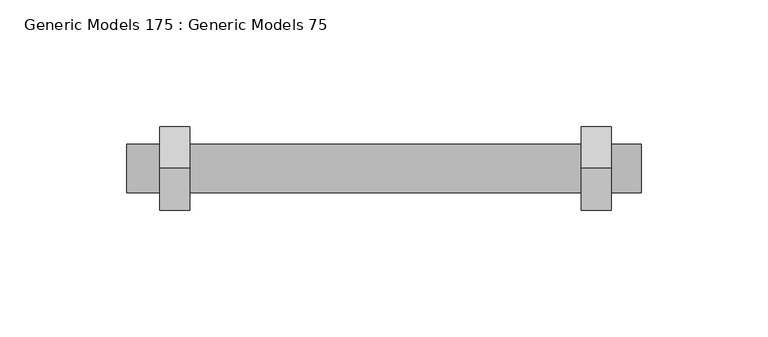
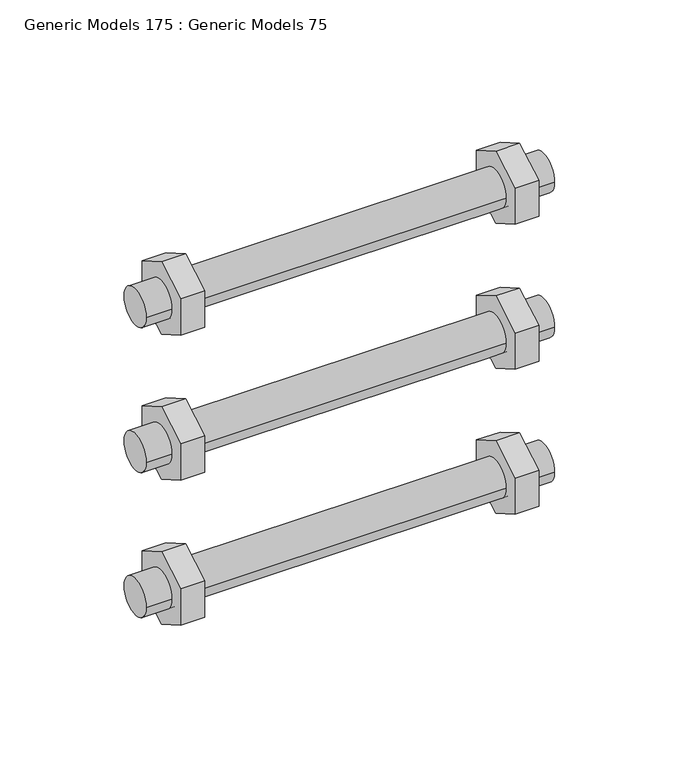
"""IFC4 building model written with IfcOpenShell, lengths in millimetres: proxy geometry, Generic Models 175 : Generic Models 75."""

import ifcopenshell
import ifcopenshell.guid

model = None  # the IFC model being written
_history = None  # IfcOwnerHistory: only IFC2X3 demands one
_inside = {}  # id of a spatial element -> (the spatial element, [elements in it])
_under = {}  # id of a project, library or spatial element -> (it, [spatial elements below it])
_declared = {}  # id of a project -> (the project, [libraries it declares])
_typed = {}  # id of a type object -> (the type object, [elements of that type])
_made_of = {}  # id of a material, layer set ... -> (it, [elements and type objects made of it])


def new_model(schema):
    """Start an empty IFC model of exactly this schema.

    Asked for "IFC4X3", IfcOpenShell would pick the latest addendum, in which some entities
    have other attributes; the version numbers below select the first issue.
    IFC2X3 requires an IfcOwnerHistory on every rooted entity: one is made here for all.
    """
    global model, _history
    if schema == "IFC4X3":
        model = ifcopenshell.file(schema_version=(4, 3, 0, 0))
    else:
        model = ifcopenshell.file(schema=schema)
    _inside.clear()
    _under.clear()
    _declared.clear()
    _typed.clear()
    _made_of.clear()
    _history = None
    if model.schema == "IFC2X3":
        org = make("IfcOrganization", Name="unknown")
        user = make(
            "IfcPersonAndOrganization",
            ThePerson=make("IfcPerson", FamilyName="unknown"),
            TheOrganization=org,
        )
        app = make(
            "IfcApplication",
            ApplicationDeveloper=org,
            Version="unknown",
            ApplicationFullName="unknown",
            ApplicationIdentifier="unknown",
        )
        _history = make(
            "IfcOwnerHistory",
            OwningUser=user,
            OwningApplication=app,
            ChangeAction="ADDED",
            CreationDate=0,
        )
    return model


def make(cls, **values):
    """One entity of the class cls with the attributes given. An attribute that is None is left unset."""
    return model.create_entity(
        cls, **{name: value for name, value in values.items() if value is not None}
    )


def rooted(cls, **values):
    """An entity with a GlobalId (a new one), such as an element, a storey or a relation."""
    return make(cls, GlobalId=ifcopenshell.guid.new(), OwnerHistory=_history, **values)


def si_unit(unit_type, name, prefix=None):
    """IfcSIUnit, for example si_unit("LENGTHUNIT", "METRE", prefix="MILLI")."""
    return make("IfcSIUnit", UnitType=unit_type, Prefix=prefix, Name=name)


def assignment(units):
    """IfcUnitAssignment: the units of a project."""
    return None if units is None else make("IfcUnitAssignment", Units=units)


def point(xyz):
    """IfcCartesianPoint."""
    return None if xyz is None else make("IfcCartesianPoint", Coordinates=xyz)


def direction(xyz):
    """IfcDirection."""
    return None if xyz is None else make("IfcDirection", DirectionRatios=xyz)


def frame(location, z_axis=None, x_axis=None):
    """IfcAxis2Placement3D, a coordinate frame: its origin and axes. An axis left out is left unset."""
    return make(
        "IfcAxis2Placement3D",
        Location=point(location),
        Axis=direction(z_axis),
        RefDirection=direction(x_axis),
    )


def frame_2d(location, x_axis=None):
    """IfcAxis2Placement2D, a coordinate frame in the plane: its origin and x axis."""
    return make(
        "IfcAxis2Placement2D", Location=point(location), RefDirection=direction(x_axis)
    )


def origin():
    """The frame at (0, 0, 0) with its axes left unset."""
    return frame((0.0, 0.0, 0.0))


def place(relative_to, where):
    """IfcLocalPlacement: puts the frame where relative to a parent placement (None: the world)."""
    return make(
        "IfcLocalPlacement", PlacementRelTo=relative_to, RelativePlacement=where
    )


def context(
    kind, dimensions, precision=None, world=None, true_north=None, identifier=None
):
    """IfcGeometricRepresentationContext, for example the 3D "Model" context."""
    return make(
        "IfcGeometricRepresentationContext",
        ContextIdentifier=identifier,
        ContextType=kind,
        CoordinateSpaceDimension=dimensions,
        Precision=precision,
        WorldCoordinateSystem=world,
        TrueNorth=true_north,
    )


def project(units=None, contexts=None):
    """IfcProject with its units and contexts."""
    return rooted(
        "IfcProject",
        Name="project",
        RepresentationContexts=contexts,
        UnitsInContext=assignment(units),
    )


def spatial(cls, under=None, at=None, **own):
    """A site, building, storey or space (cls), placed at a placement, below another one or the project."""
    s = rooted(cls, ObjectPlacement=at, **own)
    if under is not None:
        _under.setdefault(under.id(), (under, []))[1].append(s)
    return s


def polyline(points):
    """IfcPolyline through the points."""
    return make("IfcPolyline", Points=[point(p) for p in points])


def circle_curve(where, radius):
    """IfcCircle in the frame where."""
    return make("IfcCircle", Position=where, Radius=radius)


def trimmed(basis, trim1, trim2, sense, master):
    """IfcTrimmedCurve: the piece of a basis curve between two trims."""
    return make(
        "IfcTrimmedCurve",
        BasisCurve=basis,
        Trim1=trim1,
        Trim2=trim2,
        SenseAgreement=sense,
        MasterRepresentation=master,
    )


def segment(curve, same_sense, transition):
    """IfcCompositeCurveSegment."""
    return make(
        "IfcCompositeCurveSegment",
        Transition=transition,
        SameSense=same_sense,
        ParentCurve=curve,
    )


def composite_curve(segments, self_intersect=None):
    """IfcCompositeCurve: segments joined end to end."""
    return make("IfcCompositeCurve", Segments=segments, SelfIntersect=self_intersect)


def outline(outer, holes=None, kind="AREA"):
    """IfcArbitraryClosedProfileDef: a profile drawn as a closed curve; with holes, ...WithVoids."""
    if holes is None:
        return make("IfcArbitraryClosedProfileDef", ProfileType=kind, OuterCurve=outer)
    return make(
        "IfcArbitraryProfileDefWithVoids",
        ProfileType=kind,
        OuterCurve=outer,
        InnerCurves=holes,
    )


def extrude(swept, where, along, depth):
    """IfcExtrudedAreaSolid: the profile swept, set in the frame where, extruded along a direction by depth."""
    return make(
        "IfcExtrudedAreaSolid",
        SweptArea=swept,
        Position=where,
        ExtrudedDirection=direction(along),
        Depth=depth,
    )


def shape(context_of_items, identifier, shape_type, items):
    """IfcShapeRepresentation: the items that make up one representation, for example the "Body"."""
    return make(
        "IfcShapeRepresentation",
        ContextOfItems=context_of_items,
        RepresentationIdentifier=identifier,
        RepresentationType=shape_type,
        Items=items,
    )


def source(mapping_origin, context_of_items, identifier, shape_type, items):
    """IfcRepresentationMap: a shape defined once, which mapped items show again and again."""
    return make(
        "IfcRepresentationMap",
        MappingOrigin=mapping_origin,
        MappedRepresentation=shape(context_of_items, identifier, shape_type, items),
    )


def transform(
    local_origin,
    x_axis=None,
    y_axis=None,
    z_axis=None,
    scale=None,
    scale2=None,
    scale3=None,
    uniform=True,
):
    """IfcCartesianTransformationOperator3D, or its non-uniform kind. x_axis, y_axis, z_axis: its Axis1, 2, 3."""
    if uniform:
        return make(
            "IfcCartesianTransformationOperator3D",
            Axis1=direction(x_axis),
            Axis2=direction(y_axis),
            LocalOrigin=point(local_origin),
            Scale=scale,
            Axis3=direction(z_axis),
        )
    return make(
        "IfcCartesianTransformationOperator3DnonUniform",
        Axis1=direction(x_axis),
        Axis2=direction(y_axis),
        LocalOrigin=point(local_origin),
        Scale=scale,
        Axis3=direction(z_axis),
        Scale2=scale2,
        Scale3=scale3,
    )


def mapped(mapping_source, mapping_target):
    """IfcMappedItem: shows the shape of a source again, moved by a transform."""
    return make(
        "IfcMappedItem", MappingSource=mapping_source, MappingTarget=mapping_target
    )


def made_of(thing, what):
    """Note that an element or type object is made of a material, layer set ...; save() writes the relation."""
    if what is not None:
        _made_of.setdefault(what.id(), (what, []))[1].append(thing)
    return thing


def element(
    cls,
    number,
    at=None,
    inside=None,
    cuts=None,
    type_object=None,
    material=None,
    context=None,
    identifier="Body",
    shape_type=None,
    held_by="IfcProductDefinitionShape",
    body=None,
    shapes=None,
    **own,
):
    """One element of the class cls, such as IfcWall. Its Tag is "e" and its number.

    at: its placement. inside: the storey or other place that contains it. cuts: it is an
    opening in that element (IfcRelVoidsElement). A single representation is given by context,
    identifier, shape_type and body (its items); several are given by shapes. held_by: the class
    of the entity that holds the representations. save() writes the other relations.
    """
    e = rooted(cls, Tag="e%d" % number, ObjectPlacement=at, **own)
    if body is not None:
        shapes = [shape(context, identifier, shape_type, body)]
    if shapes is not None:
        e.Representation = make(held_by, Representations=shapes)
    if inside is not None:
        _inside.setdefault(inside.id(), (inside, []))[1].append(e)
    if cuts is not None:
        rooted(
            "IfcRelVoidsElement", RelatingBuildingElement=cuts, RelatedOpeningElement=e
        )
    if type_object is not None:
        _typed.setdefault(type_object.id(), (type_object, []))[1].append(e)
    return made_of(e, material)


def aggregate(whole, parts):
    """IfcRelAggregates: a whole, such as a stair, and the parts it consists of."""
    return rooted("IfcRelAggregates", RelatingObject=whole, RelatedObjects=parts)


def save(model, path):
    """Write the relations noted so far, then the file.

    IfcRelAggregates (storeys below a building ...), IfcRelContainedInSpatialStructure (elements
    in a storey), IfcRelDefinesByType, IfcRelAssociatesMaterial and IfcRelDeclares: one each for
    every whole, place, type object, material and project.
    """
    for whole, parts in _under.values():
        aggregate(whole, parts)
    for where, things in _inside.values():
        rooted(
            "IfcRelContainedInSpatialStructure",
            RelatedElements=things,
            RelatingStructure=where,
        )
    for kind, things in _typed.values():
        rooted("IfcRelDefinesByType", RelatedObjects=things, RelatingType=kind)
    for what, things in _made_of.values():
        rooted("IfcRelAssociatesMaterial", RelatedObjects=things, RelatingMaterial=what)
    for by, libraries in _declared.values():
        rooted("IfcRelDeclares", RelatingContext=by, RelatedDefinitions=libraries)
    model.write(path)


def generic_models_175_generic_models_75_7ebaa3f2(model_context):
    return source(origin(), model_context, "Body", "SweptSolid", [
        extrude(outline(polyline([(30896.7491273, 271852.097122), (30913.2469112, 271861.622122), (30929.7446951, 271852.097122), (30929.7446951, 271833.047122), (30913.2469112, 271823.522122), (30896.7491273, 271833.047122), (30896.7491273, 271852.097122)])), frame((31918.2596032, 0.0, 0.0), z_axis=(1.0, 0.0, 0.0), x_axis=(0.0, 1.0, 0.0)), (0.0, 0.0, 1.0), 11.90625),
        extrude(outline(polyline([(30896.7491273, 271775.897122), (30913.2469112, 271785.422122), (30929.7446951, 271775.897122), (30929.7446951, 271756.847122), (30913.2469112, 271747.322122), (30896.7491273, 271756.847122), (30896.7491273, 271775.897122)])), frame((31918.2596032, 0.0, 0.0), z_axis=(1.0, 0.0, 0.0), x_axis=(0.0, 1.0, 0.0)), (0.0, 0.0, 1.0), 11.90625),
        extrude(outline(polyline([(30896.7491273, 271699.697122), (30913.2469112, 271709.222122), (30929.7446951, 271699.697122), (30929.7446951, 271680.647122), (30913.2469112, 271671.122122), (30896.7491273, 271680.647122), (30896.7491273, 271699.697122)])), frame((31918.2596032, 0.0, 0.0), z_axis=(1.0, 0.0, 0.0), x_axis=(0.0, 1.0, 0.0)), (0.0, 0.0, 1.0), 11.90625),
        extrude(outline(polyline([(30896.7491273, 271852.097122), (30913.2469112, 271861.622122), (30929.7446951, 271852.097122), (30929.7446951, 271833.047122), (30913.2469112, 271823.522122), (30896.7491273, 271833.047122), (30896.7491273, 271852.097122)])), frame((31751.9689782, 0.0, 0.0), z_axis=(1.0, 0.0, 0.0), x_axis=(0.0, 1.0, 0.0)), (0.0, 0.0, 1.0), 11.90625),
        extrude(outline(polyline([(30896.7491273, 271775.897122), (30913.2469112, 271785.422122), (30929.7446951, 271775.897122), (30929.7446951, 271756.847122), (30913.2469112, 271747.322122), (30896.7491273, 271756.847122), (30896.7491273, 271775.897122)])), frame((31751.9689782, 0.0, 0.0), z_axis=(1.0, 0.0, 0.0), x_axis=(0.0, 1.0, 0.0)), (0.0, 0.0, 1.0), 11.90625),
        extrude(outline(polyline([(30896.7491273, 271699.697122), (30913.2469112, 271709.222122), (30929.7446951, 271699.697122), (30929.7446951, 271680.647122), (30913.2469112, 271671.122122), (30896.7491273, 271680.647122), (30896.7491273, 271699.697122)])), frame((31751.9689782, 0.0, 0.0), z_axis=(1.0, 0.0, 0.0), x_axis=(0.0, 1.0, 0.0)), (0.0, 0.0, 1.0), 11.90625),
        extrude(outline(composite_curve([segment(trimmed(circle_curve(frame_2d((30913.2469112, 271766.372122)), 9.525), [point((30922.7719112, 271766.372122))], [point((30903.7219112, 271766.372122))], False, "CARTESIAN"), True, "CONTINUOUS"), segment(trimmed(circle_curve(frame_2d((30913.2469112, 271766.372122)), 9.525), [point((30903.7219112, 271766.372122))], [point((30922.7719112, 271766.372122))], False, "CARTESIAN"), True, "CONTINUOUS")], self_intersect=False)), frame((31738.8721032, 0.0, 0.0), z_axis=(1.0, 0.0, 0.0), x_axis=(0.0, 1.0, 0.0)), (0.0, 0.0, 1.0), 203.2),
        extrude(outline(composite_curve([segment(trimmed(circle_curve(frame_2d((30913.2469112, 271690.172122)), 9.525), [point((30922.7719112, 271690.172122))], [point((30903.7219112, 271690.172122))], False, "CARTESIAN"), True, "CONTINUOUS"), segment(trimmed(circle_curve(frame_2d((30913.2469112, 271690.172122)), 9.525), [point((30903.7219112, 271690.172122))], [point((30922.7719112, 271690.172122))], False, "CARTESIAN"), True, "CONTINUOUS")], self_intersect=False)), frame((31738.8721032, 0.0, 0.0), z_axis=(1.0, 0.0, 0.0), x_axis=(0.0, 1.0, 0.0)), (0.0, 0.0, 1.0), 203.2),
        extrude(outline(composite_curve([segment(trimmed(circle_curve(frame_2d((30913.2469112, 271842.572122)), 9.525), [point((30922.7719112, 271842.572122))], [point((30903.7219112, 271842.572122))], False, "CARTESIAN"), True, "CONTINUOUS"), segment(trimmed(circle_curve(frame_2d((30913.2469112, 271842.572122)), 9.525), [point((30903.7219112, 271842.572122))], [point((30922.7719112, 271842.572122))], False, "CARTESIAN"), True, "CONTINUOUS")], self_intersect=False)), frame((31738.8721032, 0.0, 0.0), z_axis=(1.0, 0.0, 0.0), x_axis=(0.0, 1.0, 0.0)), (0.0, 0.0, 1.0), 203.2),
    ])


if __name__ == "__main__":
    model = new_model("IFC4")
    model_context = context("Model", 3, world=origin())
    ifc_project = project(units=[si_unit("LENGTHUNIT", "METRE", prefix="MILLI")], contexts=[model_context])
    site = spatial("IfcSite", under=ifc_project)
    building = spatial("IfcBuilding", under=site)
    placement = place(None, origin())
    generic_models_175_generic_models_75_shape = generic_models_175_generic_models_75_7ebaa3f2(model_context)
    element("IfcBuildingElementProxy", 1, Name="Generic Models 175 : Generic Models 75", ObjectType="Generic Models 175 : Generic Models 75", at=placement, inside=building, context=model_context, shape_type="MappedRepresentation", body=[
        mapped(generic_models_175_generic_models_75_shape, transform((0.0, 0.0, 0.0), x_axis=(1.0, 0.0, 0.0), y_axis=(0.0, 1.0, 0.0), z_axis=(0.0, 0.0, 1.0))),
    ])
    save(model, "model.ifc")
